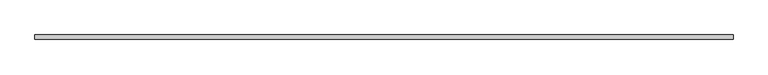
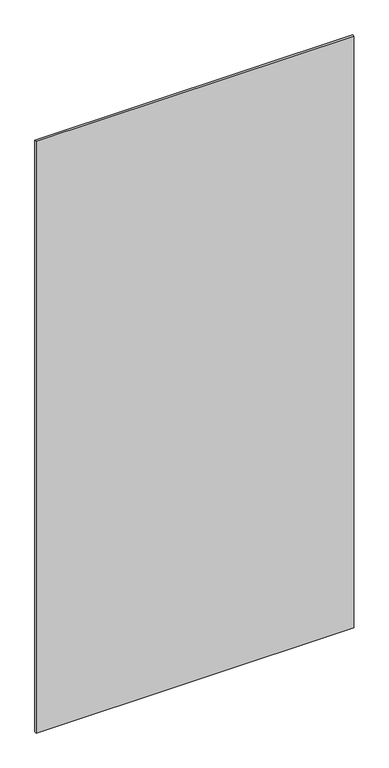
"""IFC4 building model written with IfcOpenShell, lengths in millimetres: proxy geometry, Panel:Panel:300402:Panel:300402 : Panel:Panel:300402:300124:Panel:300402:Panel:300402 : Panel:Panel:300402:300124 : Panel:Panel:300402:Panel:300402 : Panel:Panel:300402:300124:7 : Panel:Panel:300402:Panel:300402 : Panel:Panel:300402:300124:Panel:300402:Panel:300402 : Panel:Panel:300402:300124 : Panel:Panel:300402:Panel:300402 : Panel:Panel:300402:300124:300083."""

from ifc_helpers import new_model, si_unit, frame, origin, place, context, project, spatial, polyline, outline, extrude, source, transform, mapped, element, save


def generic_models_3b43eac6(model_context):
    return source(origin(), model_context, "Body", "SweptSolid", [
        extrude(outline(polyline([(569227.0867239, -579076.8913841), (570446.2867239, -579076.8913841), (570446.2867239, -579084.8288841), (569227.0867239, -579084.8288841), (569227.0867239, -579076.8913841)])), frame((0.0, 0.0, 3733.8), z_axis=(0.0, 0.0, 1.0), x_axis=(1.0, 0.0, 0.0)), (0.0, 0.0, 1.0), 2400.3),
    ])


if __name__ == "__main__":
    model = new_model("IFC4")
    model_context = context("Model", 3, world=origin())
    ifc_project = project(units=[si_unit("LENGTHUNIT", "METRE", prefix="MILLI")], contexts=[model_context])
    site = spatial("IfcSite", under=ifc_project)
    building = spatial("IfcBuilding", under=site)
    placement = place(None, origin())
    generic_models_shape = generic_models_3b43eac6(model_context)
    element("IfcBuildingElementProxy", 1, Name="Panel:Panel:300402:Panel:300402 : Panel:Panel:300402:300124:Panel:300402:Panel:300402 : Panel:Panel:300402:300124 : Panel:Panel:300402:Panel:300402 : Panel:Panel:300402:300124:7 : Panel:Panel:300402:Panel:300402 : Panel:Panel:300402:300124:Panel:300402:Panel:300402 : Panel:Panel:300402:300124 : Panel:Panel:300402:Panel:300402 : Panel:Panel:300402:300124:300083", ObjectType="Panel:Panel:300402:Panel:300402 : Panel:Panel:300402:300124:Panel:300402:Panel:300402 : Panel:Panel:300402:300124 : Panel:Panel:300402:Panel:300402 : Panel:Panel:300402:300124:7 : Panel:Panel:300402:Panel:300402 : Panel:Panel:300402:300124:Panel:300402:Panel:300402 : Panel:Panel:300402:300124 : Panel:Panel:300402:Panel:300402 : Panel:Panel:300402:300124:300083", at=placement, inside=building, context=model_context, shape_type="MappedRepresentation", body=[
        mapped(generic_models_shape, transform((0.0, 0.0, 0.0), x_axis=(1.0, 0.0, 0.0), y_axis=(0.0, 1.0, 0.0), z_axis=(0.0, 0.0, 1.0))),
    ])
    save(model, "model.ifc")

# Revit data of these elements
# Type "Panel:Panel:300402:Panel:300402 : Panel:Panel:300402:300124:Panel:300402:Panel:300402 : Panel:Panel:300402:300124 : Panel:Panel:300402:Panel:300402 : Panel:Panel:300402:300124:7 : Panel:Panel:300402:Panel:300402 : Panel:Panel:300402:300124:Panel:300402:Panel:300402 : Panel:Panel:300402:300124 : Panel:Panel:300402:Panel:300402 : Panel:Panel:300402:300124:300083"
#   NameOverride = "Panel:Panel:300402:Panel:300402 : Panel:Panel:300402:300124:Panel:300402:Panel:300402 : Panel:Panel:300402:300124 : Panel:Panel:300402:Panel:300402 : Panel:Panel:300402:300124:300083"
#   ObjectTypeOverride = "Panel:300402:Panel:300402 : Panel:Panel:300402:300124 : Panel:Panel:300402:Panel:300402 : Panel:Panel:300402:300124"
#   Reference = "Panel"
#   Tag = "300083"
# Element 1 (IfcBuildingElementProxy, "Panel:Panel:300402:Panel:300402 : Panel:Panel:300402:300124:Panel:300402:Panel:300402 : Panel:Panel:300402:300124 : Panel:Panel:300402:Panel:300402 : Panel:Panel:300402:300124:7 : Panel:Panel:300402:Panel:300402 : Panel:Panel:300402:300124:Panel:300402:Panel:300402 : Panel:Panel:300402:300124 : Panel:Panel:300402:Panel:300402 : Panel:Panel:300402:300124:300083")
#   Materials on its faces: "5/16\" PHENOLIC RESIN PANELS (CLASS A FLAME SPREAD) - EXPOSED FASTENERS"
# Materials
#   "5/16\" PHENOLIC RESIN PANELS (CLASS A FLAME SPREAD) - EXPOSED FASTENERS": class "Unassigned", colour RGB 64 64 64, transparency 0, Keynote = "M07420000.01", Cost = 0
